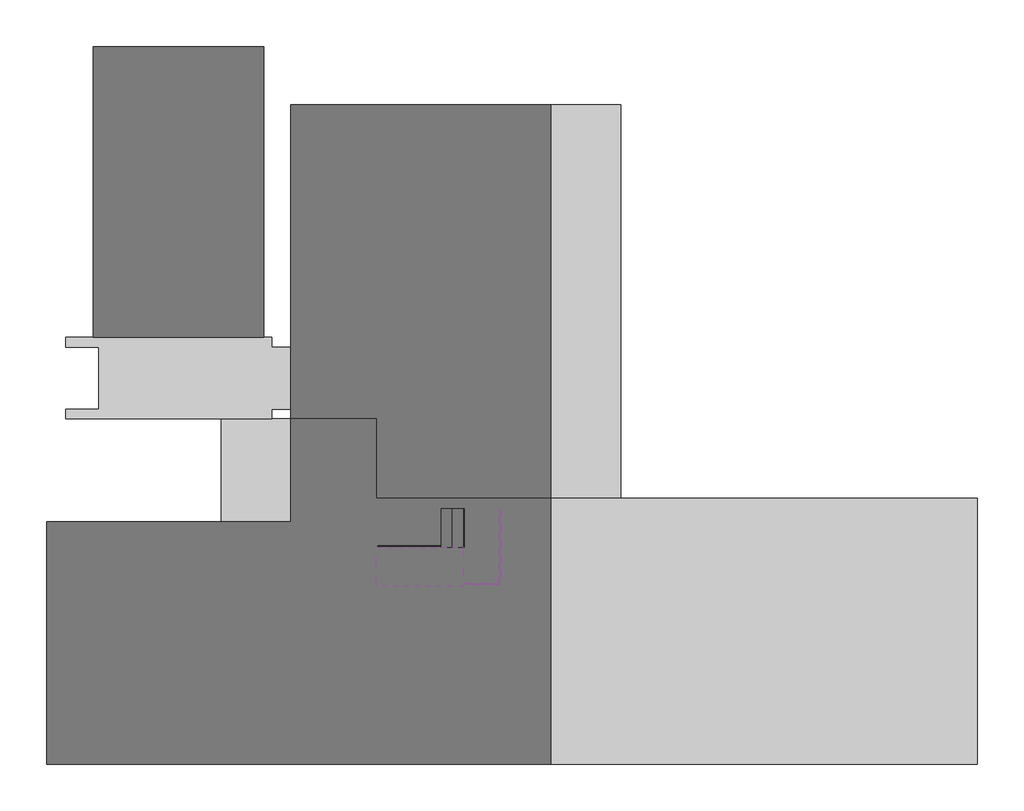
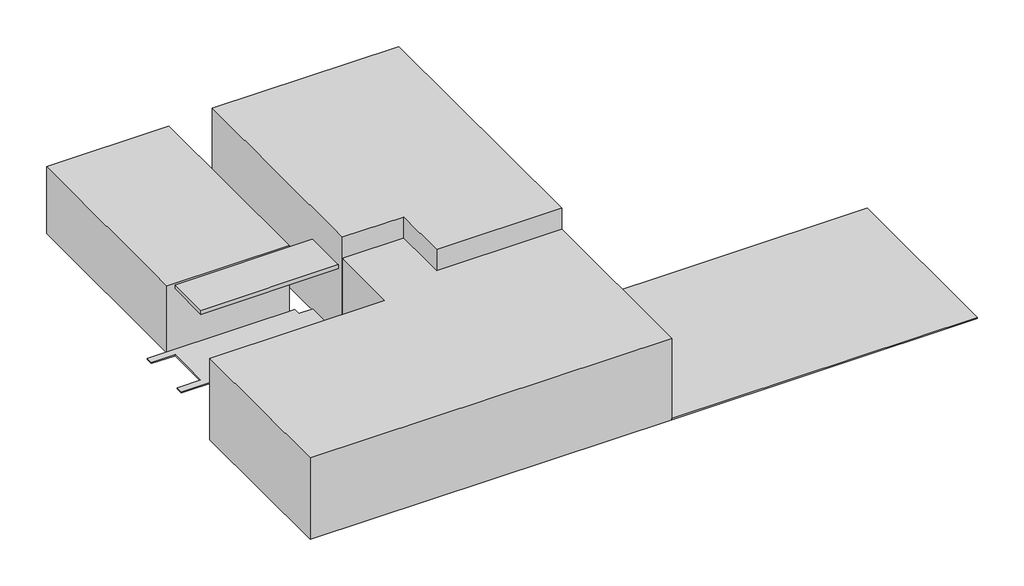
# One storey: 7 proxies, 6 railings, 2 stair flights, 1 slab.
"""IFC4 building model written with IfcOpenShell, lengths in millimetres."""

import ifcopenshell
import ifcopenshell.guid

model = None  # the IFC model being written
_history = None  # IfcOwnerHistory: only IFC2X3 demands one
_inside = {}  # id of a spatial element -> (the spatial element, [elements in it])
_under = {}  # id of a project, library or spatial element -> (it, [spatial elements below it])
_declared = {}  # id of a project -> (the project, [libraries it declares])
_typed = {}  # id of a type object -> (the type object, [elements of that type])
_made_of = {}  # id of a material, layer set ... -> (it, [elements and type objects made of it])


def new_model(schema):
    """Start an empty IFC model of exactly this schema.

    Asked for "IFC4X3", IfcOpenShell would pick the latest addendum, in which some entities
    have other attributes; the version numbers below select the first issue.
    IFC2X3 requires an IfcOwnerHistory on every rooted entity: one is made here for all.
    """
    global model, _history
    if schema == "IFC4X3":
        model = ifcopenshell.file(schema_version=(4, 3, 0, 0))
    else:
        model = ifcopenshell.file(schema=schema)
    _inside.clear()
    _under.clear()
    _declared.clear()
    _typed.clear()
    _made_of.clear()
    _history = None
    if model.schema == "IFC2X3":
        org = make("IfcOrganization", Name="unknown")
        user = make(
            "IfcPersonAndOrganization",
            ThePerson=make("IfcPerson", FamilyName="unknown"),
            TheOrganization=org,
        )
        app = make(
            "IfcApplication",
            ApplicationDeveloper=org,
            Version="unknown",
            ApplicationFullName="unknown",
            ApplicationIdentifier="unknown",
        )
        _history = make(
            "IfcOwnerHistory",
            OwningUser=user,
            OwningApplication=app,
            ChangeAction="ADDED",
            CreationDate=0,
        )
    return model


def make(cls, **values):
    """One entity of the class cls with the attributes given. An attribute that is None is left unset."""
    return model.create_entity(
        cls, **{name: value for name, value in values.items() if value is not None}
    )


def rooted(cls, **values):
    """An entity with a GlobalId (a new one), such as an element, a storey or a relation."""
    return make(cls, GlobalId=ifcopenshell.guid.new(), OwnerHistory=_history, **values)


def si_unit(unit_type, name, prefix=None):
    """IfcSIUnit, for example si_unit("LENGTHUNIT", "METRE", prefix="MILLI")."""
    return make("IfcSIUnit", UnitType=unit_type, Prefix=prefix, Name=name)


def assignment(units):
    """IfcUnitAssignment: the units of a project."""
    return None if units is None else make("IfcUnitAssignment", Units=units)


def point(xyz):
    """IfcCartesianPoint."""
    return None if xyz is None else make("IfcCartesianPoint", Coordinates=xyz)


def direction(xyz):
    """IfcDirection."""
    return None if xyz is None else make("IfcDirection", DirectionRatios=xyz)


def frame(location, z_axis=None, x_axis=None):
    """IfcAxis2Placement3D, a coordinate frame: its origin and axes. An axis left out is left unset."""
    return make(
        "IfcAxis2Placement3D",
        Location=point(location),
        Axis=direction(z_axis),
        RefDirection=direction(x_axis),
    )


def origin():
    """The frame at (0, 0, 0) with its axes left unset."""
    return frame((0.0, 0.0, 0.0))


def place(relative_to, where):
    """IfcLocalPlacement: puts the frame where relative to a parent placement (None: the world)."""
    return make(
        "IfcLocalPlacement", PlacementRelTo=relative_to, RelativePlacement=where
    )


def context(
    kind, dimensions, precision=None, world=None, true_north=None, identifier=None
):
    """IfcGeometricRepresentationContext, for example the 3D "Model" context."""
    return make(
        "IfcGeometricRepresentationContext",
        ContextIdentifier=identifier,
        ContextType=kind,
        CoordinateSpaceDimension=dimensions,
        Precision=precision,
        WorldCoordinateSystem=world,
        TrueNorth=true_north,
    )


def project(units=None, contexts=None):
    """IfcProject with its units and contexts."""
    return rooted(
        "IfcProject",
        Name="project",
        RepresentationContexts=contexts,
        UnitsInContext=assignment(units),
    )


def spatial(cls, under=None, at=None, **own):
    """A site, building, storey or space (cls), placed at a placement, below another one or the project."""
    s = rooted(cls, ObjectPlacement=at, **own)
    if under is not None:
        _under.setdefault(under.id(), (under, []))[1].append(s)
    return s


def polyline(points):
    """IfcPolyline through the points."""
    return make("IfcPolyline", Points=[point(p) for p in points])


def outline(outer, holes=None, kind="AREA"):
    """IfcArbitraryClosedProfileDef: a profile drawn as a closed curve; with holes, ...WithVoids."""
    if holes is None:
        return make("IfcArbitraryClosedProfileDef", ProfileType=kind, OuterCurve=outer)
    return make(
        "IfcArbitraryProfileDefWithVoids",
        ProfileType=kind,
        OuterCurve=outer,
        InnerCurves=holes,
    )


def extrude(swept, where, along, depth):
    """IfcExtrudedAreaSolid: the profile swept, set in the frame where, extruded along a direction by depth."""
    return make(
        "IfcExtrudedAreaSolid",
        SweptArea=swept,
        Position=where,
        ExtrudedDirection=direction(along),
        Depth=depth,
    )


def faces_of(points, faces, orient=None, outer=None):
    """IfcFace entities. A face is a list of loops; a loop is a list of indices into points, from 0.

    orient and outer hold one flag for each loop. By default every Orientation is true, the
    first loop of a face is its IfcFaceOuterBound and the others are IfcFaceBound.
    """
    made = []
    for i, loops in enumerate(faces):
        bounds = []
        for j, loop in enumerate(loops):
            is_outer = j == 0 if outer is None else outer[i][j]
            bounds.append(
                make(
                    "IfcFaceOuterBound" if is_outer else "IfcFaceBound",
                    Bound=make("IfcPolyLoop", Polygon=[points[k] for k in loop]),
                    Orientation=True if orient is None else orient[i][j],
                )
            )
        made.append(make("IfcFace", Bounds=bounds))
    return made


def faceted_brep(points, faces, orient=None, outer=None, voids=None):
    """IfcFacetedBrep: a solid bounded by flat faces; with voids (closed shells), ...WithVoids."""
    shared = [point(p) for p in points]
    hull = make("IfcClosedShell", CfsFaces=faces_of(shared, faces, orient, outer))
    if voids is None:
        return make("IfcFacetedBrep", Outer=hull)
    return make(
        "IfcFacetedBrepWithVoids",
        Outer=hull,
        Voids=[
            make(cls, CfsFaces=faces_of(shared, fs, o, b)) for cls, fs, o, b in voids
        ],
    )


def shape(context_of_items, identifier, shape_type, items):
    """IfcShapeRepresentation: the items that make up one representation, for example the "Body"."""
    return make(
        "IfcShapeRepresentation",
        ContextOfItems=context_of_items,
        RepresentationIdentifier=identifier,
        RepresentationType=shape_type,
        Items=items,
    )


def source(mapping_origin, context_of_items, identifier, shape_type, items):
    """IfcRepresentationMap: a shape defined once, which mapped items show again and again."""
    return make(
        "IfcRepresentationMap",
        MappingOrigin=mapping_origin,
        MappedRepresentation=shape(context_of_items, identifier, shape_type, items),
    )


def transform(
    local_origin,
    x_axis=None,
    y_axis=None,
    z_axis=None,
    scale=None,
    scale2=None,
    scale3=None,
    uniform=True,
):
    """IfcCartesianTransformationOperator3D, or its non-uniform kind. x_axis, y_axis, z_axis: its Axis1, 2, 3."""
    if uniform:
        return make(
            "IfcCartesianTransformationOperator3D",
            Axis1=direction(x_axis),
            Axis2=direction(y_axis),
            LocalOrigin=point(local_origin),
            Scale=scale,
            Axis3=direction(z_axis),
        )
    return make(
        "IfcCartesianTransformationOperator3DnonUniform",
        Axis1=direction(x_axis),
        Axis2=direction(y_axis),
        LocalOrigin=point(local_origin),
        Scale=scale,
        Axis3=direction(z_axis),
        Scale2=scale2,
        Scale3=scale3,
    )


def mapped(mapping_source, mapping_target):
    """IfcMappedItem: shows the shape of a source again, moved by a transform."""
    return make(
        "IfcMappedItem", MappingSource=mapping_source, MappingTarget=mapping_target
    )


def made_of(thing, what):
    """Note that an element or type object is made of a material, layer set ...; save() writes the relation."""
    if what is not None:
        _made_of.setdefault(what.id(), (what, []))[1].append(thing)
    return thing


def element(
    cls,
    number,
    at=None,
    inside=None,
    cuts=None,
    type_object=None,
    material=None,
    context=None,
    identifier="Body",
    shape_type=None,
    held_by="IfcProductDefinitionShape",
    body=None,
    shapes=None,
    **own,
):
    """One element of the class cls, such as IfcWall. Its Tag is "e" and its number.

    at: its placement. inside: the storey or other place that contains it. cuts: it is an
    opening in that element (IfcRelVoidsElement). A single representation is given by context,
    identifier, shape_type and body (its items); several are given by shapes. held_by: the class
    of the entity that holds the representations. save() writes the other relations.
    """
    e = rooted(cls, Tag="e%d" % number, ObjectPlacement=at, **own)
    if body is not None:
        shapes = [shape(context, identifier, shape_type, body)]
    if shapes is not None:
        e.Representation = make(held_by, Representations=shapes)
    if inside is not None:
        _inside.setdefault(inside.id(), (inside, []))[1].append(e)
    if cuts is not None:
        rooted(
            "IfcRelVoidsElement", RelatingBuildingElement=cuts, RelatedOpeningElement=e
        )
    if type_object is not None:
        _typed.setdefault(type_object.id(), (type_object, []))[1].append(e)
    return made_of(e, material)


def aggregate(whole, parts):
    """IfcRelAggregates: a whole, such as a stair, and the parts it consists of."""
    return rooted("IfcRelAggregates", RelatingObject=whole, RelatedObjects=parts)


def save(model, path):
    """Write the relations noted so far, then the file.

    IfcRelAggregates (storeys below a building ...), IfcRelContainedInSpatialStructure (elements
    in a storey), IfcRelDefinesByType, IfcRelAssociatesMaterial and IfcRelDeclares: one each for
    every whole, place, type object, material and project.
    """
    for whole, parts in _under.values():
        aggregate(whole, parts)
    for where, things in _inside.values():
        rooted(
            "IfcRelContainedInSpatialStructure",
            RelatedElements=things,
            RelatingStructure=where,
        )
    for kind, things in _typed.values():
        rooted("IfcRelDefinesByType", RelatedObjects=things, RelatingType=kind)
    for what, things in _made_of.values():
        rooted("IfcRelAssociatesMaterial", RelatedObjects=things, RelatingMaterial=what)
    for by, libraries in _declared.values():
        rooted("IfcRelDeclares", RelatingContext=by, RelatedDefinitions=libraries)
    model.write(path)


def railing_81dbcb3b(model_context):
    return source(origin(), model_context, "Body", "SweptSolid", [
        extrude(outline(polyline([(1832.4523952, 3702.0), (1832.4523952, 3594.0), (1856.4523952, 3594.0), (1856.4523952, 3702.0), (1866.9523952, 3702.0), (1866.9523952, 3700.0), (1858.4523952, 3700.0), (1858.4523952, 3592.0), (1830.4523952, 3592.0), (1830.4523952, 3700.0), (1821.9523952, 3700.0), (1821.9523952, 3702.0), (1832.4523952, 3702.0)])), frame((-12226.1487231, 0.0, 0.0), z_axis=(1.0, 0.0, 0.0), x_axis=(0.0, 1.0, 0.0)), (0.0, 0.0, 1.0), 1940.0),
    ])


def railing_0d959ca4(model_context):
    return source(origin(), model_context, "Body", "SweptSolid", [
        extrude(outline(polyline([(-4674.5702584, 2133.3602771), (-4674.5702584, 2121.3602771), (-6610.5702584, 2121.3602771), (-6610.5702584, 2133.3602771), (-4674.5702584, 2133.3602771)])), frame((0.0, 0.0, 4122.0679199), z_axis=(0.0, 0.0, 1.0), x_axis=(1.0, 0.0, 0.0)), (0.0, 0.0, 1.0), 1100.0),
    ])


def railing_24874f95(model_context):
    return source(origin(), model_context, "Body", "SweptSolid", [
        extrude(outline(polyline([(1832.4523952, 3702.0), (1832.4523952, 3594.0), (1856.4523952, 3594.0), (1856.4523952, 3702.0), (1866.9523952, 3702.0), (1866.9523952, 3700.0), (1858.4523952, 3700.0), (1858.4523952, 3592.0), (1830.4523952, 3592.0), (1830.4523952, 3700.0), (1821.9523952, 3700.0), (1821.9523952, 3702.0), (1832.4523952, 3702.0)])), frame((-12226.1487231, 0.0, 0.0), z_axis=(1.0, 0.0, 0.0), x_axis=(0.0, 1.0, 0.0)), (0.0, 0.0, 1.0), 925.0),
    ])


def railing_29f9e2f6(model_context):
    return source(origin(), model_context, "Body", "SweptSolid", [
        extrude(outline(polyline([(-4674.5702584, 2133.3602771), (-4674.5702584, 2121.3602771), (-5595.5702584, 2121.3602771), (-5595.5702584, 2133.3602771), (-4674.5702584, 2133.3602771)])), frame((0.0, 0.0, 4122.0679199), z_axis=(0.0, 0.0, 1.0), x_axis=(1.0, 0.0, 0.0)), (0.0, 0.0, 1.0), 1100.0),
    ])


def railing_c44cfcee(model_context):
    return source(origin(), model_context, "Body", "SweptSolid", [
        extrude(outline(polyline([(1672.2222222, -4460.281307), (500.0, -4460.281307), (1877.7777778, -2220.281307), (3050.0, -2220.281307), (1672.2222222, -4460.281307)])), frame((0.0, -5573.3699847, 0.0), z_axis=(0.0, 1.0, 0.0), x_axis=(0.0, 0.0, 1.0)), (0.0, 0.0, 1.0), 12.0),
    ])


model = new_model("IFC4")

# Units and contexts
model_context = context("Model", 3, world=origin())
ifc_project = project(units=[si_unit("LENGTHUNIT", "METRE", prefix="MILLI")], contexts=[model_context])

# Site, building, storey
site = spatial("IfcSite", under=ifc_project)
building = spatial("IfcBuilding", under=site)
storey = spatial("IfcBuildingStorey", under=building, Name="PAVIMENTO TÉRREO", Elevation=500.0)

# Proxies
placement = place(None, origin())
element("IfcBuildingElementProxy", 1, Name="GARAGEM : GARAGEM", ObjectType="GARAGEM : GARAGEM", at=placement, inside=storey, context=model_context, shape_type="SweptSolid", body=[
    extrude(outline(polyline([(-7360.281307, 7304.4300153), (-7360.281307, -195.5699847), (-11760.281307, -195.5699847), (-11760.281307, 7304.4300153), (-7360.281307, 7304.4300153)])), frame((0.0, 0.0, 500.0), z_axis=(0.0, 0.0, 1.0), x_axis=(1.0, 0.0, 0.0)), (0.0, 0.0, 1.0), 2550.0),
])
element("IfcBuildingElementProxy", 2, Name="PERGOLADO SALAS : PERGOLADO SALAS", ObjectType="PERGOLADO SALAS : PERGOLADO SALAS", at=placement, inside=storey, context=model_context, shape_type="SweptSolid", body=[
    extrude(outline(polyline([(1839.718693, 5804.4300153), (1839.718693, -4345.5699847), (39.718693, -4345.5699847), (39.718693, 5804.4300153), (1839.718693, 5804.4300153)])), frame((0.0, 0.0, 500.0), z_axis=(0.0, 0.0, 1.0), x_axis=(1.0, 0.0, 0.0)), (0.0, 0.0, 1.0), 50.0),
])
element("IfcBuildingElementProxy", 3, Name="VARANDA GOURMET : VARANDA GOURMET", ObjectType="VARANDA GOURMET : VARANDA GOURMET", at=placement, inside=storey, context=model_context, shape_type="SweptSolid", body=[
    extrude(outline(polyline([(11039.718693, -4345.5699847), (11039.718693, -11195.5699847), (39.718693, -11195.5699847), (39.718693, -4345.5699847), (11039.718693, -4345.5699847)])), frame((0.0, 0.0, 500.0), z_axis=(0.0, 0.0, 1.0), x_axis=(1.0, 0.0, 0.0)), (0.0, 0.0, 1.0), 50.0),
])
element("IfcBuildingElementProxy", 4, Name="PÓRTICO ENTRADA : PÓRTICO ENTRADA", ObjectType="PÓRTICO ENTRADA : PÓRTICO ENTRADA", at=placement, inside=storey, context=model_context, shape_type="SweptSolid", body=[
    extrude(outline(polyline([(-7160.281307, -445.5699847), (-6660.281307, -445.5699847), (-6660.281307, -2045.5699847), (-7160.281307, -2045.5699847), (-7160.281307, -2295.5699847), (-12460.281307, -2295.5699847), (-12460.281307, -2045.5699847), (-11610.281307, -2045.5699847), (-11610.281307, -445.5699847), (-12460.281307, -445.5699847), (-12460.281307, -195.5699847), (-7160.281307, -195.5699847), (-7160.281307, -445.5699847)])), frame((0.0, 0.0, 500.0), z_axis=(0.0, 0.0, 1.0), x_axis=(1.0, 0.0, 0.0)), (0.0, 0.0, 1.0), 50.0),
    extrude(outline(polyline([(-6660.281307, -445.5699847), (-6660.281307, -2045.5699847), (-11610.281307, -2045.5699847), (-11610.281307, -445.5699847), (-6660.281307, -445.5699847)])), frame((0.0, 0.0, 3050.0), z_axis=(0.0, 0.0, 1.0), x_axis=(1.0, 0.0, 0.0)), (0.0, 0.0, 1.0), 150.0),
])
element("IfcBuildingElementProxy", 5, Name="SALAS : SALAS", ObjectType="SALAS : SALAS", at=placement, inside=storey, context=model_context, shape_type="SweptSolid", body=[
    extrude(outline(polyline([(39.718693, 5804.4300153), (39.718693, -4345.5699847), (-4460.281307, -4345.5699847), (-4460.281307, -2295.5699847), (-6660.281307, -2295.5699847), (-6660.281307, 5804.4300153), (39.718693, 5804.4300153)])), frame((0.0, 0.0, 500.0), z_axis=(0.0, 0.0, 1.0), x_axis=(1.0, 0.0, 0.0)), (0.0, 0.0, 1.0), 3900.0),
])
element("IfcBuildingElementProxy", 6, Name="PROJEÇÃO : PROJEÇÃO", ObjectType="PROJEÇÃO : PROJEÇÃO", at=placement, inside=storey, context=model_context, shape_type="SweptSolid", body=[
    extrude(outline(polyline([(-6660.281307, -2295.5699847), (-6660.281307, -4945.5699847), (-8460.281307, -4945.5699847), (-8460.281307, -2295.5699847), (-6660.281307, -2295.5699847)])), frame((0.0, 0.0, 500.0), z_axis=(0.0, 0.0, 1.0), x_axis=(1.0, 0.0, 0.0)), (0.0, 0.0, 1.0), 50.0),
])
element("IfcBuildingElementProxy", 7, Name="COZINHA E LAVANDERIA : COZINHA E LAVANDERIA", ObjectType="COZINHA E LAVANDERIA : COZINHA E LAVANDERIA", at=placement, inside=storey, context=model_context, shape_type="SweptSolid", body=[
    extrude(outline(polyline([(-4460.281307, -4345.5699847), (39.718693, -4345.5699847), (39.718693, -11195.5699847), (-12960.281307, -11195.5699847), (-12960.281307, -4945.5699847), (-6660.281307, -4945.5699847), (-6660.281307, -2295.5699847), (-4460.281307, -2295.5699847), (-4460.281307, -4345.5699847)])), frame((0.0, 0.0, 500.0), z_axis=(0.0, 0.0, 1.0), x_axis=(1.0, 0.0, 0.0)), (0.0, 0.0, 1.0), 3100.0),
])

# Railings
railing_shape = railing_81dbcb3b(model_context)
element("IfcRailing", 8, ObjectType="ML_Perfil U de embutir3 : ML_Perfil U de embutir", at=placement, inside=storey, context=model_context, shape_type="MappedRepresentation", body=[
    mapped(railing_shape, transform((-3117.2337022, -16861.5187078, -1650.0), x_axis=(0.0, -1.0, 0.0), y_axis=(1.0, 0.0, 0.0), z_axis=(0.0, 0.0, 1.0))),
])
railing_2_shape = railing_0d959ca4(model_context)
element("IfcRailing", 9, ObjectType="ML_Painéis3 : ML_Painéis", at=placement, inside=storey, context=model_context, shape_type="MappedRepresentation", body=[
    mapped(railing_2_shape, transform((-3400.141584, -11247.9402431, -2172.0679199), x_axis=(0.0, -1.0, 0.0), y_axis=(1.0, 0.0, 0.0), z_axis=(0.0, 0.0, 1.0))),
])
railing_3_shape = railing_24874f95(model_context)
element("IfcRailing", 10, ObjectType="ML_Perfil U de embutir4 : ML_Perfil U de embutir", at=placement, inside=storey, context=model_context, shape_type="MappedRepresentation", body=[
    mapped(railing_3_shape, transform((10005.8674161, -8397.3223799, -1650.0), x_axis=(1.0, 0.0, 0.0), y_axis=(0.0, 1.0, 0.0), z_axis=(0.0, 0.0, 1.0))),
])
railing_4_shape = railing_29f9e2f6(model_context)
element("IfcRailing", 11, ObjectType="ML_Painéis4 : ML_Painéis", at=placement, inside=storey, context=model_context, shape_type="MappedRepresentation", body=[
    mapped(railing_4_shape, transform((3377.2889515, -8680.2302618, -2172.0679199), x_axis=(1.0, 0.0, 0.0), y_axis=(0.0, 1.0, 0.0), z_axis=(0.0, 0.0, 1.0))),
])
railing_5_shape = railing_c44cfcee(model_context)
element("IfcRailing", 12, ObjectType="ML_Guarda_corpo lance : ML_Guarda_corpo lance", at=placement, inside=storey, context=model_context, shape_type="MappedRepresentation", body=[
    mapped(railing_5_shape, transform((0.0, 0.0, 0.0), x_axis=(1.0, 0.0, 0.0), y_axis=(0.0, 1.0, 0.0), z_axis=(0.0, 0.0, 1.0))),
])
element("IfcRailing", 13, ObjectType="ML_Guarda_corpo lance1 : ML_Guarda_corpo lance", at=placement, inside=storey, context=model_context, shape_type="MappedRepresentation", body=[
    mapped(railing_5_shape, transform((0.0, 0.0, 0.0), x_axis=(1.0, 0.0, 0.0), y_axis=(0.0, 1.0, 0.0), z_axis=(0.0, 0.0, 1.0))),
])

# Slab
element("IfcSlab", 14, ObjectType="Espessura de 300 mm", at=placement, inside=storey, context=model_context, shape_type="SolidModel", body=[
    faceted_brep([(-2220.281307, -4605.3699847, 2030.0), (-2220.281307, -5605.3699847, 2030.0), (-2220.281307, -6605.3699847, 2030.0), (-2018.8487302, -6605.3699847, 2030.0), (-1220.281307, -6605.3699847, 2030.0), (-1220.281307, -4605.3699847, 2030.0), (-2141.7138837, -4605.3699847, 2030.0), (-2220.281307, -4605.3699847, 1857.7777778), (-2220.281307, -4605.3699847, 1681.6747992), (-2220.281307, -5605.3699847, 1681.6747992), (-2220.281307, -5605.3699847, 1853.8970214), (-2220.281307, -6605.3699847, 1853.8970214), (-2018.8487302, -6605.3699847, 1730.0), (-1220.281307, -6605.3699847, 1730.0), (-1220.281307, -4605.3699847, 1730.0), (-2141.7138837, -4605.3699847, 1730.0), (-2018.8487302, -5605.3699847, 1730.0), (-2141.7138837, -5605.3699847, 1730.0), (-2141.7138837, -5605.3699847, 1805.5718206)], [[[0, 1, 2, 3, 4, 5, 6]], [[1, 0, 7, 8, 9, 10]], [[2, 1, 10, 11]], [[2, 11, 12, 13, 4, 3]], [[5, 4, 13, 14]], [[8, 7, 0, 6, 5, 14, 15]], [[16, 17, 15, 14, 13, 12]], [[17, 16, 18]], [[15, 17, 9, 8]], [[17, 18, 10, 9]], [[16, 12, 11, 10, 18]]]),
    extrude(outline(polyline([(-2220.281307, -4605.3699847), (-1220.281307, -4605.3699847), (-1220.281307, -6605.3699847), (-2220.281307, -6605.3699847), (-2220.281307, -5605.3699847), (-2220.281307, -4605.3699847)])), frame((0.0, 0.0, 2030.0), z_axis=(0.0, 0.0, 1.0), x_axis=(1.0, 0.0, 0.0)), (0.0, 0.0, 1.0), 20.0),
])

# Stair flights
element("IfcStairFlight", 15, ObjectType="Profundidade de 150 mm - SEM BOCEL", at=placement, inside=storey, context=model_context, shape_type="SolidModel", body=[
    faceted_brep([(-4180.281307, -4605.3699847, 652.2222222), (-4460.281307, -4605.3699847, 652.2222222), (-4460.281307, -5605.3699847, 652.2222222), (-4180.281307, -5605.3699847, 652.2222222), (-4180.281307, -4605.3699847, 500.0), (-4460.281307, -4605.3699847, 500.0), (-4460.281307, -5605.3699847, 500.0), (-4180.281307, -5605.3699847, 500.0), (-3900.281307, -4605.3699847, 824.4444444), (-4180.281307, -4605.3699847, 824.4444444), (-4180.281307, -5605.3699847, 824.4444444), (-3900.281307, -5605.3699847, 824.4444444), (-3900.281307, -4605.3699847, 648.3414658), (-4141.4558192, -4605.3699847, 500.0), (-4141.4558192, -5605.3699847, 500.0), (-3900.281307, -5605.3699847, 648.3414658), (-3620.281307, -4605.3699847, 996.6666667), (-3900.281307, -4605.3699847, 996.6666667), (-3900.281307, -5605.3699847, 996.6666667), (-3620.281307, -5605.3699847, 996.6666667), (-3620.281307, -4605.3699847, 820.5636881), (-3620.281307, -5605.3699847, 820.5636881), (-3340.281307, -4605.3699847, 1168.8888889), (-3620.281307, -4605.3699847, 1168.8888889), (-3620.281307, -5605.3699847, 1168.8888889), (-3340.281307, -5605.3699847, 1168.8888889), (-3340.281307, -4605.3699847, 992.7859103), (-3340.281307, -5605.3699847, 992.7859103), (-3060.281307, -4605.3699847, 1341.1111111), (-3340.281307, -4605.3699847, 1341.1111111), (-3340.281307, -5605.3699847, 1341.1111111), (-3060.281307, -5605.3699847, 1341.1111111), (-3060.281307, -4605.3699847, 1165.0081325), (-3060.281307, -5605.3699847, 1165.0081325), (-2780.281307, -4605.3699847, 1513.3333333), (-3060.281307, -4605.3699847, 1513.3333333), (-3060.281307, -5605.3699847, 1513.3333333), (-2780.281307, -5605.3699847, 1513.3333333), (-2780.281307, -4605.3699847, 1337.2303547), (-2780.281307, -5605.3699847, 1337.2303547), (-2500.281307, -4605.3699847, 1685.5555556), (-2780.281307, -4605.3699847, 1685.5555556), (-2780.281307, -5605.3699847, 1685.5555556), (-2500.281307, -5605.3699847, 1685.5555556), (-2500.281307, -4605.3699847, 1509.452577), (-2500.281307, -5605.3699847, 1509.452577), (-2220.281307, -4605.3699847, 1857.7777778), (-2500.281307, -4605.3699847, 1857.7777778), (-2500.281307, -5605.3699847, 1857.7777778), (-2220.281307, -5605.3699847, 1857.7777778), (-2220.281307, -4605.3699847, 1681.6747992), (-2220.281307, -5605.3699847, 1681.6747992), (-2220.281307, -5605.3699847, 1853.8970214)], [[[0, 1, 2, 3]], [[1, 0, 4, 5]], [[2, 1, 5, 6]], [[3, 2, 6, 7]], [[8, 9, 10, 11]], [[4, 0, 9, 8, 12, 13]], [[0, 3, 10, 9]], [[3, 7, 14, 15, 11, 10]], [[16, 17, 18, 19]], [[17, 16, 20, 12, 8]], [[8, 11, 18, 17]], [[19, 18, 11, 15, 21]], [[22, 23, 24, 25]], [[23, 22, 26, 20, 16]], [[16, 19, 24, 23]], [[25, 24, 19, 21, 27]], [[28, 29, 30, 31]], [[29, 28, 32, 26, 22]], [[22, 25, 30, 29]], [[31, 30, 25, 27, 33]], [[34, 35, 36, 37]], [[35, 34, 38, 32, 28]], [[28, 31, 36, 35]], [[37, 36, 31, 33, 39]], [[40, 41, 42, 43]], [[41, 40, 44, 38, 34]], [[34, 37, 42, 41]], [[43, 42, 37, 39, 45]], [[46, 47, 48, 49]], [[47, 46, 50, 44, 40]], [[40, 43, 48, 47]], [[49, 48, 43, 45, 51, 52]], [[46, 49, 52, 51, 50]], [[5, 4, 13, 14, 7, 6]], [[14, 13, 12, 20, 26, 32, 38, 44, 50, 51, 45, 39, 33, 27, 21, 15]]]),
    extrude(outline(polyline([(-4180.281307, -4605.3699847), (-4180.281307, -5605.3699847), (-4460.281307, -5605.3699847), (-4460.281307, -4605.3699847), (-4180.281307, -4605.3699847)])), frame((0.0, 0.0, 652.2222222), z_axis=(0.0, 0.0, 1.0), x_axis=(1.0, 0.0, 0.0)), (0.0, 0.0, 1.0), 20.0),
    extrude(outline(polyline([(-3900.281307, -4605.3699847), (-3900.281307, -5605.3699847), (-4180.281307, -5605.3699847), (-4180.281307, -4605.3699847), (-3900.281307, -4605.3699847)])), frame((0.0, 0.0, 824.4444444), z_axis=(0.0, 0.0, 1.0), x_axis=(1.0, 0.0, 0.0)), (0.0, 0.0, 1.0), 20.0),
    extrude(outline(polyline([(-3620.281307, -4605.3699847), (-3620.281307, -5605.3699847), (-3900.281307, -5605.3699847), (-3900.281307, -4605.3699847), (-3620.281307, -4605.3699847)])), frame((0.0, 0.0, 996.6666667), z_axis=(0.0, 0.0, 1.0), x_axis=(1.0, 0.0, 0.0)), (0.0, 0.0, 1.0), 20.0),
    extrude(outline(polyline([(-3340.281307, -4605.3699847), (-3340.281307, -5605.3699847), (-3620.281307, -5605.3699847), (-3620.281307, -4605.3699847), (-3340.281307, -4605.3699847)])), frame((0.0, 0.0, 1168.8888889), z_axis=(0.0, 0.0, 1.0), x_axis=(1.0, 0.0, 0.0)), (0.0, 0.0, 1.0), 20.0),
    extrude(outline(polyline([(-3060.281307, -4605.3699847), (-3060.281307, -5605.3699847), (-3340.281307, -5605.3699847), (-3340.281307, -4605.3699847), (-3060.281307, -4605.3699847)])), frame((0.0, 0.0, 1341.1111111), z_axis=(0.0, 0.0, 1.0), x_axis=(1.0, 0.0, 0.0)), (0.0, 0.0, 1.0), 20.0),
    extrude(outline(polyline([(-2780.281307, -4605.3699847), (-2780.281307, -5605.3699847), (-3060.281307, -5605.3699847), (-3060.281307, -4605.3699847), (-2780.281307, -4605.3699847)])), frame((0.0, 0.0, 1513.3333333), z_axis=(0.0, 0.0, 1.0), x_axis=(1.0, 0.0, 0.0)), (0.0, 0.0, 1.0), 20.0),
    extrude(outline(polyline([(-2500.281307, -4605.3699847), (-2500.281307, -5605.3699847), (-2780.281307, -5605.3699847), (-2780.281307, -4605.3699847), (-2500.281307, -4605.3699847)])), frame((0.0, 0.0, 1685.5555556), z_axis=(0.0, 0.0, 1.0), x_axis=(1.0, 0.0, 0.0)), (0.0, 0.0, 1.0), 20.0),
    extrude(outline(polyline([(-2220.281307, -4605.3699847), (-2220.281307, -5605.3699847), (-2500.281307, -5605.3699847), (-2500.281307, -4605.3699847), (-2220.281307, -4605.3699847)])), frame((0.0, 0.0, 1857.7777778), z_axis=(0.0, 0.0, 1.0), x_axis=(1.0, 0.0, 0.0)), (0.0, 0.0, 1.0), 20.0),
])
element("IfcStairFlight", 16, ObjectType="Profundidade de 150 mm - SEM BOCEL", at=placement, inside=storey, context=model_context, shape_type="SolidModel", body=[
    faceted_brep([(-2500.281307, -6605.3699847, 2202.2222222), (-2220.281307, -6605.3699847, 2202.2222222), (-2220.281307, -5605.3699847, 2202.2222222), (-2500.281307, -5605.3699847, 2202.2222222), (-2500.281307, -6605.3699847, 2026.1192436), (-2220.281307, -6605.3699847, 1853.8970214), (-2220.281307, -6605.3699847, 2030.0), (-2220.281307, -5605.3699847, 1853.8970214), (-2500.281307, -5605.3699847, 2026.1192436), (-2780.281307, -6605.3699847, 2374.4444444), (-2500.281307, -6605.3699847, 2374.4444444), (-2500.281307, -5605.3699847, 2374.4444444), (-2780.281307, -5605.3699847, 2374.4444444), (-2780.281307, -6605.3699847, 2198.3414658), (-2780.281307, -5605.3699847, 2198.3414658), (-3060.281307, -6605.3699847, 2546.6666667), (-2780.281307, -6605.3699847, 2546.6666667), (-2780.281307, -5605.3699847, 2546.6666667), (-3060.281307, -5605.3699847, 2546.6666667), (-3060.281307, -6605.3699847, 2370.5636881), (-3060.281307, -5605.3699847, 2370.5636881), (-3340.281307, -6605.3699847, 2718.8888889), (-3060.281307, -6605.3699847, 2718.8888889), (-3060.281307, -5605.3699847, 2718.8888889), (-3340.281307, -5605.3699847, 2718.8888889), (-3340.281307, -6605.3699847, 2542.7859103), (-3340.281307, -5605.3699847, 2542.7859103), (-3620.281307, -6605.3699847, 2891.1111111), (-3340.281307, -6605.3699847, 2891.1111111), (-3340.281307, -5605.3699847, 2891.1111111), (-3620.281307, -5605.3699847, 2891.1111111), (-3620.281307, -6605.3699847, 2715.0081325), (-3620.281307, -5605.3699847, 2715.0081325), (-3900.281307, -6605.3699847, 3063.3333333), (-3620.281307, -6605.3699847, 3063.3333333), (-3620.281307, -5605.3699847, 3063.3333333), (-3900.281307, -5605.3699847, 3063.3333333), (-3900.281307, -6605.3699847, 2887.2303547), (-3900.281307, -5605.3699847, 2887.2303547), (-4180.281307, -6605.3699847, 3235.5555556), (-3900.281307, -6605.3699847, 3235.5555556), (-3900.281307, -5605.3699847, 3235.5555556), (-4180.281307, -5605.3699847, 3235.5555556), (-4180.281307, -6605.3699847, 3059.452577), (-4180.281307, -5605.3699847, 3059.452577), (-4460.281307, -6605.3699847, 3407.7777778), (-4180.281307, -6605.3699847, 3407.7777778), (-4180.281307, -5605.3699847, 3407.7777778), (-4460.281307, -5605.3699847, 3407.7777778), (-4460.281307, -6605.3699847, 3231.6747992), (-4460.281307, -5605.3699847, 3231.6747992)], [[[0, 1, 2, 3]], [[1, 0, 4, 5, 6]], [[2, 1, 6, 5, 7]], [[3, 2, 7, 8]], [[9, 10, 11, 12]], [[10, 9, 13, 4, 0]], [[11, 10, 0, 3]], [[12, 11, 3, 8, 14]], [[15, 16, 17, 18]], [[16, 15, 19, 13, 9]], [[17, 16, 9, 12]], [[18, 17, 12, 14, 20]], [[21, 22, 23, 24]], [[22, 21, 25, 19, 15]], [[23, 22, 15, 18]], [[24, 23, 18, 20, 26]], [[27, 28, 29, 30]], [[28, 27, 31, 25, 21]], [[29, 28, 21, 24]], [[30, 29, 24, 26, 32]], [[33, 34, 35, 36]], [[34, 33, 37, 31, 27]], [[35, 34, 27, 30]], [[36, 35, 30, 32, 38]], [[39, 40, 41, 42]], [[40, 39, 43, 37, 33]], [[41, 40, 33, 36]], [[42, 41, 36, 38, 44]], [[45, 46, 47, 48]], [[46, 45, 49, 43, 39]], [[47, 46, 39, 42]], [[48, 47, 42, 44, 50]], [[45, 48, 50, 49]], [[5, 4, 13, 19, 25, 31, 37, 43, 49, 50, 44, 38, 32, 26, 20, 14, 8, 7]]]),
    extrude(outline(polyline([(-2500.281307, -6605.3699847), (-2500.281307, -5605.3699847), (-2220.281307, -5605.3699847), (-2220.281307, -6605.3699847), (-2500.281307, -6605.3699847)])), frame((0.0, 0.0, 2202.2222222), z_axis=(0.0, 0.0, 1.0), x_axis=(1.0, 0.0, 0.0)), (0.0, 0.0, 1.0), 20.0),
    extrude(outline(polyline([(-2780.281307, -6605.3699847), (-2780.281307, -5605.3699847), (-2500.281307, -5605.3699847), (-2500.281307, -6605.3699847), (-2780.281307, -6605.3699847)])), frame((0.0, 0.0, 2374.4444444), z_axis=(0.0, 0.0, 1.0), x_axis=(1.0, 0.0, 0.0)), (0.0, 0.0, 1.0), 20.0),
    extrude(outline(polyline([(-3060.281307, -6605.3699847), (-3060.281307, -5605.3699847), (-2780.281307, -5605.3699847), (-2780.281307, -6605.3699847), (-3060.281307, -6605.3699847)])), frame((0.0, 0.0, 2546.6666667), z_axis=(0.0, 0.0, 1.0), x_axis=(1.0, 0.0, 0.0)), (0.0, 0.0, 1.0), 20.0),
    extrude(outline(polyline([(-3340.281307, -6605.3699847), (-3340.281307, -5605.3699847), (-3060.281307, -5605.3699847), (-3060.281307, -6605.3699847), (-3340.281307, -6605.3699847)])), frame((0.0, 0.0, 2718.8888889), z_axis=(0.0, 0.0, 1.0), x_axis=(1.0, 0.0, 0.0)), (0.0, 0.0, 1.0), 20.0),
    extrude(outline(polyline([(-3620.281307, -6605.3699847), (-3620.281307, -5605.3699847), (-3340.281307, -5605.3699847), (-3340.281307, -6605.3699847), (-3620.281307, -6605.3699847)])), frame((0.0, 0.0, 2891.1111111), z_axis=(0.0, 0.0, 1.0), x_axis=(1.0, 0.0, 0.0)), (0.0, 0.0, 1.0), 20.0),
    extrude(outline(polyline([(-3900.281307, -6605.3699847), (-3900.281307, -5605.3699847), (-3620.281307, -5605.3699847), (-3620.281307, -6605.3699847), (-3900.281307, -6605.3699847)])), frame((0.0, 0.0, 3063.3333333), z_axis=(0.0, 0.0, 1.0), x_axis=(1.0, 0.0, 0.0)), (0.0, 0.0, 1.0), 20.0),
    extrude(outline(polyline([(-4180.281307, -6605.3699847), (-4180.281307, -5605.3699847), (-3900.281307, -5605.3699847), (-3900.281307, -6605.3699847), (-4180.281307, -6605.3699847)])), frame((0.0, 0.0, 3235.5555556), z_axis=(0.0, 0.0, 1.0), x_axis=(1.0, 0.0, 0.0)), (0.0, 0.0, 1.0), 20.0),
    extrude(outline(polyline([(-4460.281307, -6605.3699847), (-4460.281307, -5605.3699847), (-4180.281307, -5605.3699847), (-4180.281307, -6605.3699847), (-4460.281307, -6605.3699847)])), frame((0.0, 0.0, 3407.7777778), z_axis=(0.0, 0.0, 1.0), x_axis=(1.0, 0.0, 0.0)), (0.0, 0.0, 1.0), 20.0),
])

save(model, "model.ifc")

# Revit data of these elements
# Type "ML_Perfil U de embutir3 : ML_Perfil U de embutir"
#   ME_Compr [instance default] = 1.94 m
#   ME_Material Perfil [instance default] = .ALUMÍNIO COM PINTURA ELETROSTÁTICA BRANCA
# Type "ML_Painéis3 : ML_Painéis"
#   ME_Área [instance default] = 2.1296 m²
#   ME_Espessura [instance default] = 0.012 m
#   ME_Dist Painéis [instance default] = 0.002 m
#   ME_Compr Painéis [instance default] = 1.936 m
#   ME_Compr [instance default] = 1.94 m
#   ME_Altura [instance default] = 1.10 m
#   ME_Quant Painéis [instance default] = 3
#   ME_Painel Único [instance default] = yes
#   ME_Paineis Vários [instance default] = no
#   ME_Material Tipo Vidro [instance default] = .VIDRO GENÉRICO
# Type "ML_Perfil U de embutir4 : ML_Perfil U de embutir"
#   ME_Compr [instance default] = 0.925 m
#   ME_Material Perfil [instance default] = .ALUMÍNIO COM PINTURA ELETROSTÁTICA BRANCA
# Type "ML_Painéis4 : ML_Painéis"
#   ME_Área [instance default] = 1.0131 m²
#   ME_Espessura [instance default] = 0.012 m
#   ME_Dist Painéis [instance default] = 0.002 m
#   ME_Compr Painéis [instance default] = 0.921 m
#   ME_Compr [instance default] = 0.925 m
#   ME_Altura [instance default] = 1.10 m
#   ME_Quant Painéis [instance default] = 3
#   ME_Painel Único [instance default] = yes
#   ME_Paineis Vários [instance default] = no
#   ME_Material Tipo Vidro [instance default] = .VIDRO GENÉRICO
# Type "ML_Guarda_corpo lance : ML_Guarda_corpo lance"
#   ME_Área = 2.62578 m²
#   ME_Espessura [instance default] = 0.012 m
#   ME_Compr Painéis = 2.629804 m
#   ME_Altura = 0.998469 m
#   ME_Material Tipo Vidro [instance default] = .VIDRO GENÉRICO
# Type "ML_Guarda_corpo lance1 : ML_Guarda_corpo lance"
#   ME_Área = 2.62578 m²
#   ME_Espessura [instance default] = 0.012 m
#   ME_Compr Painéis = 2.629804 m
#   ME_Altura = 0.998469 m
#   ME_Material Tipo Vidro [instance default] = .VIDRO GENÉRICO
# Element 1 (IfcBuildingElementProxy, "GARAGEM : GARAGEM")
#   Phase Created = CC_EV
#   Materials on its faces: "Forma padrão"
# Element 2 (IfcBuildingElementProxy, "PERGOLADO SALAS : PERGOLADO SALAS")
#   Phase Created = CC_EV
#   Materials on its faces: "Forma padrão"
# Element 3 (IfcBuildingElementProxy, "VARANDA GOURMET : VARANDA GOURMET")
#   Phase Created = CC_EV
#   Materials on its faces: "Forma padrão"
# Element 4 (IfcBuildingElementProxy, "PÓRTICO ENTRADA : PÓRTICO ENTRADA")
#   Phase Created = CC_EV
#   Materials on its faces: "Forma padrão"
# Element 5 (IfcBuildingElementProxy, "SALAS : SALAS")
#   Phase Created = CC_EV
#   Materials on its faces: "Forma padrão"
# Element 6 (IfcBuildingElementProxy, "PROJEÇÃO : PROJEÇÃO")
#   Phase Created = CC_EV
#   Materials on its faces: "Forma padrão"
# Element 7 (IfcBuildingElementProxy, "COZINHA E LAVANDERIA : COZINHA E LAVANDERIA")
#   Phase Created = CC_EV
#   Materials on its faces: "Forma padrão"
# Element 8 (IfcRailing, "ML_Perfil U de embutir3 : ML_Perfil U de embutir")
#   Uso = "PATAMAR"
#   ME_Compr = 1.94 m
#   ME_Material Perfil = .ALUMÍNIO COM PINTURA ELETROSTÁTICA BRANCA
#   Phase Created = CC_AP
#   Materials on its faces: ".ALUMÍNIO COM PINTURA ELETROSTÁTICA BRANCA"
# Element 9 (IfcRailing, "ML_Painéis3 : ML_Painéis")
#   Uso = "PATAMAR"
#   ME_Área = 2.1296 m²
#   ME_Espessura = 0.012 m
#   ME_Dist Painéis = 0.002 m
#   ME_Compr Painéis = 1.936 m
#   ME_Compr = 1.94 m
#   ME_Altura = 1.10 m
#   ME_Quant Painéis = 3
#   ME_Painel Único = yes
#   ME_Paineis Vários = no
#   ME_Material Tipo Vidro = .VIDRO GENÉRICO
#   Phase Created = CC_AP
#   Materials on its faces: ".VIDRO GENÉRICO"
# Element 10 (IfcRailing, "ML_Perfil U de embutir4 : ML_Perfil U de embutir")
#   Uso = "PATAMAR"
#   ME_Compr = 0.925 m
#   ME_Material Perfil = .ALUMÍNIO COM PINTURA ELETROSTÁTICA BRANCA
#   Phase Created = CC_AP
#   Materials on its faces: ".ALUMÍNIO COM PINTURA ELETROSTÁTICA BRANCA"
# Element 11 (IfcRailing, "ML_Painéis4 : ML_Painéis")
#   Uso = "PATAMAR"
#   ME_Área = 1.0131 m²
#   ME_Espessura = 0.012 m
#   ME_Dist Painéis = 0.002 m
#   ME_Compr Painéis = 0.921 m
#   ME_Compr = 0.925 m
#   ME_Altura = 1.10 m
#   ME_Quant Painéis = 3
#   ME_Painel Único = yes
#   ME_Paineis Vários = no
#   ME_Material Tipo Vidro = .VIDRO GENÉRICO
#   Phase Created = CC_AP
#   Materials on its faces: ".VIDRO GENÉRICO"
# Element 12 (IfcRailing, "ML_Guarda_corpo lance : ML_Guarda_corpo lance")
#   Uso = "LANCE"
#   ME_Espessura = 0.012 m
#   ME_Material Tipo Vidro = .VIDRO GENÉRICO
#   Phase Created = CC_AP
#   Materials on its faces: ".VIDRO GENÉRICO"
# Element 13 (IfcRailing, "ML_Guarda_corpo lance1 : ML_Guarda_corpo lance")
#   Uso = "LANCE"
#   ME_Espessura = 0.012 m
#   ME_Material Tipo Vidro = .VIDRO GENÉRICO
#   Phase Created = CC_AP
#   Materials on its faces: ".VIDRO GENÉRICO"
# Element 14 (IfcSlab, "Espessura de 300 mm")
#   Phase Created = CC_AP
#   Materials on its faces: ".SOLEIRA DE CUMARÚ"
# Elements 15, 16 (IfcStairFlight, "Profundidade de 150 mm - SEM BOCEL")
#   Phase Created = CC_AP
#   Materials on its faces: ".SOLEIRA DE CUMARÚ", ".CONCRETO ESTRUTURAL"
# Materials
#   ".ALUMÍNIO COM PINTURA ELETROSTÁTICA BRANCA": class "CC_METAIS", colour RGB 241 241 241, transparency 0, Cost = 0
#   ".VIDRO GENÉRICO": class ".CC_VIDRO", colour RGB 0 128 192, transparency 0.9, Description = "Vidro comum", Cost = 0
#   "Forma padrão": class "Genérico", colour RGB 185 189 196, transparency 0.5, Cost = 0
#   ".SOLEIRA DE CUMARÚ": class ".CC_MADEIRAS", colour RGB 188 160 135, transparency 0, Cost = 0
#   ".CONCRETO ESTRUTURAL": class ".CC_CONCRETO", colour RGB 192 192 192, transparency 0, Description = "Concreto moldado no local", Cost = 0
